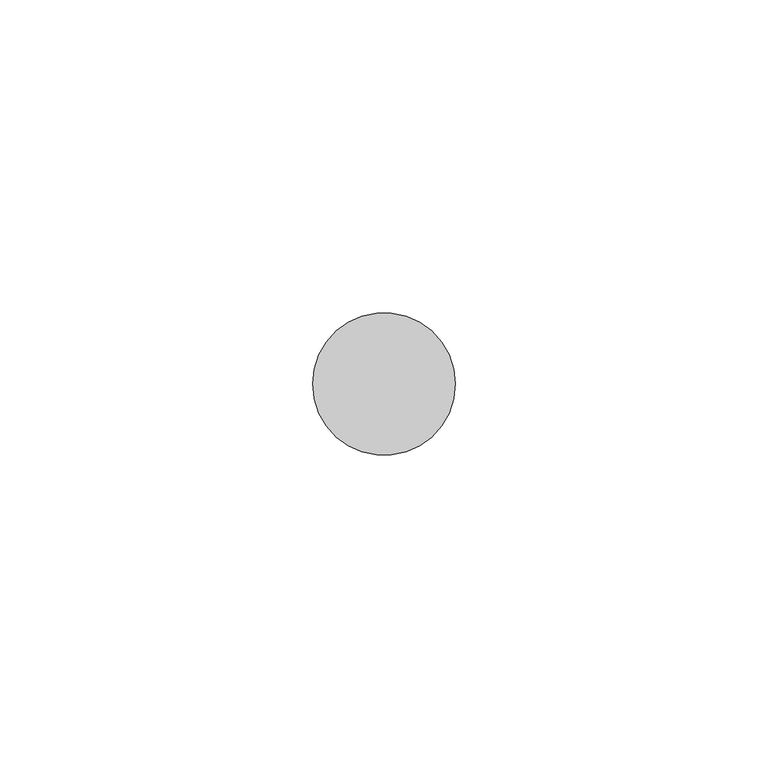
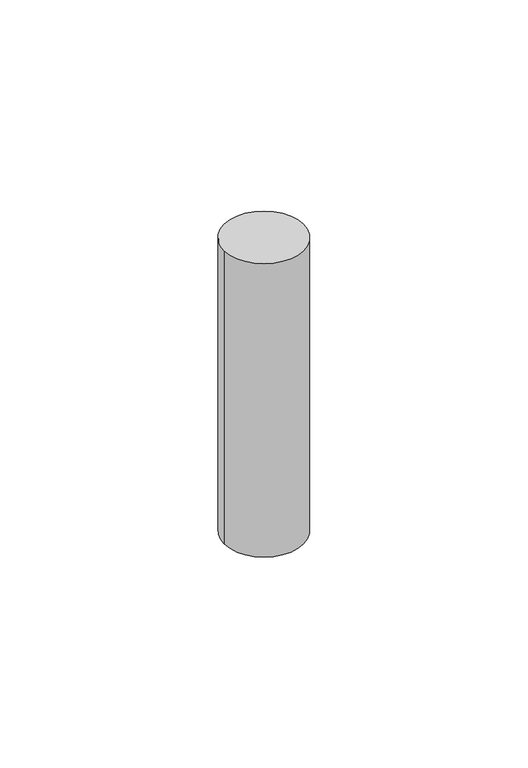
"""IFC4 building model written with IfcOpenShell, lengths in millimetres: proxy geometry, Bolt11:Bolt003:304214 : Bolt11:Bolt003:304214."""

from ifc_helpers import new_model, si_unit, point, frame, frame_2d, origin, place, context, project, spatial, circle_curve, trimmed, segment, composite_curve, outline, extrude, source, transform, mapped, element, save


def generic_models_fd5fb220(model_context):
    return source(origin(), model_context, "Body", "SweptSolid", [
        extrude(outline(composite_curve([segment(trimmed(circle_curve(frame_2d((9804.3437094, 2174.9207483)), 11.4045168), [point((9815.7482262, 2174.9207483))], [point((9792.9391926, 2174.9207483))], False, "CARTESIAN"), True, "CONTINUOUS"), segment(trimmed(circle_curve(frame_2d((9804.3437094, 2174.9207483)), 11.4045168), [point((9792.9391926, 2174.9207483))], [point((9815.7482262, 2174.9207483))], False, "CARTESIAN"), True, "CONTINUOUS")], self_intersect=False)), frame((0.0, 0.0, 36645.5959962), z_axis=(0.0, 0.0, 1.0), x_axis=(1.0, 0.0, 0.0)), (0.0, 0.0, 1.0), 88.9),
    ])


if __name__ == "__main__":
    model = new_model("IFC4")
    model_context = context("Model", 3, world=origin())
    ifc_project = project(units=[si_unit("LENGTHUNIT", "METRE", prefix="MILLI")], contexts=[model_context])
    site = spatial("IfcSite", under=ifc_project)
    building = spatial("IfcBuilding", under=site)
    placement = place(None, origin())
    generic_models_shape = generic_models_fd5fb220(model_context)
    element("IfcBuildingElementProxy", 1, Name="Bolt11:Bolt003:304214 : Bolt11:Bolt003:304214", ObjectType="Bolt11:Bolt003:304214 : Bolt11:Bolt003:304214", at=placement, inside=building, context=model_context, shape_type="MappedRepresentation", body=[
        mapped(generic_models_shape, transform((0.0, 0.0, 0.0), x_axis=(1.0, 0.0, 0.0), y_axis=(0.0, 1.0, 0.0), z_axis=(0.0, 0.0, 1.0))),
    ])
    save(model, "model.ifc")

# Revit data of these elements
# Type "Bolt11:Bolt003:304214 : Bolt11:Bolt003:304214"
#   NameOverride = "Bolt11:Bolt003:304214"
#   ObjectTypeOverride = "Bolt11:Bolt003"
#   Reference = "Bolt003"
#   Category = "Generic Models"
#   Tag = "304214"
# Element 1 (IfcBuildingElementProxy, "Bolt11:Bolt003:304214 : Bolt11:Bolt003:304214")
#   Materials on its faces: "TUBE STEEL STRINGER WELDED TO ANCHORED STEEL PLATE - SEE STRUCT DWGS"
# Materials
#   "TUBE STEEL STRINGER WELDED TO ANCHORED STEEL PLATE - SEE STRUCT DWGS": class "Unassigned", colour RGB 128 128 128, transparency 0, Cost = 0
